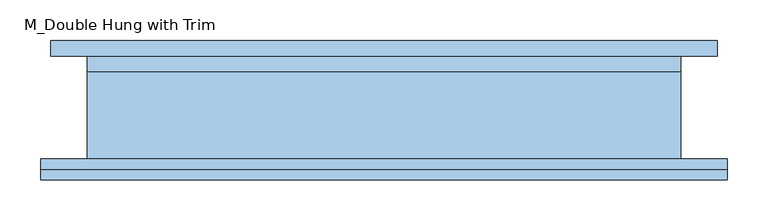
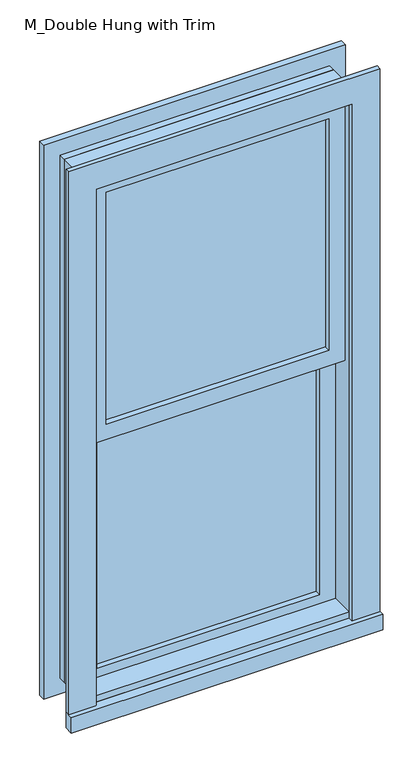
"""IFC4 building model written with IfcOpenShell, lengths in millimetres: window geometry, M_Double Hung with Trim."""

from ifc_helpers import new_model, si_unit, frame, origin, place, context, project, spatial, polyline, outline, extrude, source, transform, mapped, element, save


def m_double_hung_with_trim_aa4956d1(model_context):
    return source(origin(), model_context, "Body", "SweptSolid", [
        extrude(outline(polyline([(-301.625, 15.825), (-301.625, 28.525), (301.625, 28.525), (301.625, 15.825), (-301.625, 15.825)])), frame((0.0, 0.0, 628.65), z_axis=(0.0, 0.0, 1.0), x_axis=(1.0, 0.0, 0.0)), (0.0, 0.0, 1.0), 682.625),
        extrude(outline(polyline([(1355.725, -346.075), (584.2, -346.075), (584.2, 346.075), (1355.725, 346.075), (1355.725, -346.075)]), holes=[polyline([(1311.275, -301.625), (1311.275, 301.625), (628.65, 301.625), (628.65, -301.625), (1311.275, -301.625)])]), frame((0.0, -0.05, 0.0), z_axis=(0.0, 1.0, 0.0), x_axis=(0.0, 0.0, 1.0)), (0.0, 0.0, 1.0), 44.45),
        extrude(outline(polyline([(-422.275, -89.2), (-422.275, -63.5), (422.275, -63.5), (422.275, -89.2), (-422.275, -89.2)])), frame((0.0, 0.0, 539.75), z_axis=(0.0, 0.0, 1.0), x_axis=(1.0, 0.0, 0.0)), (0.0, 0.0, 1.0), 44.45),
        extrude(outline(polyline([(2139.95, -422.275), (539.75, -422.275), (539.75, 422.275), (2139.95, 422.275), (2139.95, -422.275)]), holes=[polyline([(2063.75, -346.075), (2063.75, 346.075), (584.2, 346.075), (584.2, -346.075), (2063.75, -346.075)])]), frame((0.0, -76.5, 0.0), z_axis=(0.0, 1.0, 0.0), x_axis=(0.0, 0.0, 1.0)), (0.0, 0.0, 1.0), 13.0),
        extrude(outline(polyline([(2127.25, 409.575), (2127.25, -409.575), (539.75, -409.575), (539.75, 409.575), (2127.25, 409.575)]), holes=[polyline([(2051.05, 333.375), (615.95, 333.375), (615.95, -333.375), (2051.05, -333.375), (2051.05, 333.375)])]), frame((0.0, 63.5, 0.0), z_axis=(0.0, 1.0, 0.0), x_axis=(0.0, 0.0, 1.0)), (0.0, 0.0, 1.0), 19.0),
        extrude(outline(polyline([(301.625, -15.925), (301.625, -28.625), (-301.625, -28.625), (-301.625, -15.925), (301.625, -15.925)])), frame((0.0, 0.0, 1355.725), z_axis=(0.0, 0.0, 1.0), x_axis=(1.0, 0.0, 0.0)), (0.0, 0.0, 1.0), 663.575),
        extrude(outline(polyline([(2063.75, -346.075), (1311.275, -346.075), (1311.275, 346.075), (2063.75, 346.075), (2063.75, -346.075)]), holes=[polyline([(2019.3, -301.625), (2019.3, 301.625), (1355.725, 301.625), (1355.725, -301.625), (2019.3, -301.625)])]), frame((0.0, -44.5, 0.0), z_axis=(0.0, 1.0, 0.0), x_axis=(0.0, 0.0, 1.0)), (0.0, 0.0, 1.0), 44.45),
        extrude(outline(polyline([(2082.8, -365.125), (584.2, -365.125), (584.2, 365.125), (2082.8, 365.125), (2082.8, -365.125)]), holes=[polyline([(2051.05, -333.375), (2051.05, 333.375), (615.95, 333.375), (615.95, -333.375), (2051.05, -333.375)])]), frame((0.0, 44.4, 0.0), z_axis=(0.0, 1.0, 0.0), x_axis=(0.0, 0.0, 1.0)), (0.0, 0.0, 1.0), 19.1),
        extrude(outline(polyline([(2082.8, 365.125), (2082.8, -365.125), (584.2, -365.125), (584.2, 365.125), (2082.8, 365.125)]), holes=[polyline([(2063.75, 346.075), (603.25, 346.075), (603.25, -346.075), (2063.75, -346.075), (2063.75, 346.075)])]), frame((0.0, -63.5, 0.0), z_axis=(0.0, 1.0, 0.0), x_axis=(0.0, 0.0, 1.0)), (0.0, 0.0, 1.0), 107.9),
    ])


if __name__ == "__main__":
    model = new_model("IFC4")
    model_context = context("Model", 3, world=origin())
    ifc_project = project(units=[si_unit("LENGTHUNIT", "METRE", prefix="MILLI")], contexts=[model_context])
    site = spatial("IfcSite", under=ifc_project)
    building = spatial("IfcBuilding", under=site)
    placement = place(None, origin())
    m_double_hung_with_trim_shape = m_double_hung_with_trim_aa4956d1(model_context)
    element("IfcWindow", 1, ObjectType="M_Double Hung with Trim : 2'  4 3/4\" x  4'  11\"", at=placement, inside=building, context=model_context, shape_type="MappedRepresentation", body=[
        mapped(m_double_hung_with_trim_shape, transform((0.0, 0.0, 0.0), x_axis=(1.0, 0.0, 0.0), y_axis=(0.0, 1.0, 0.0), z_axis=(0.0, 0.0, 1.0))),
    ])
    save(model, "model.ifc")

# Revit data of these elements
# Type "M_Double Hung with Trim : 2'  4 3/4\" x  4'  11\""
#   Type Mark = "73"
#   Construction Type Id = "GSP4R"
#   Analytic Construction = "1/8 in Pilkington single glazing"
#   Visual Light Transmittance = 0.9
#   Thermal Resistance (R) = 0.271106 (m²·K)/W
#   Solar Heat Gain Coefficient = 0.78
#   Heat Transfer Coefficient (U) = 3.6886 W/(m²·K)
#   Height = 4' - 11"
#   Default Sill Height = 1' - 11"
#   Trim Projection - Ext. = 0' - 0.51181"
#   Trim Projection - Int. = 0' - 0.74803"
#   Trim Width - Exterior = 0' - 3"
#   Trim Width - Interior = 0' - 3"
#   Width = 2' - 4 3/4"
#   Window Inset = 0' - 0.74803"
#   Glass Pane Material = EXISTING WINDOW
#   Sash = Trim
#   Trim Exterior Material = Trim
#   Trim Interior Material = Trim
#   Wall Closure = (empty or 0)
# Element 1 (IfcWindow, "M_Double Hung with Trim : 2'  4 3/4\" x  4'  11\"")
#   Materials on its faces: "Trim", "EXISTING WINDOW"
# Materials
#   "EXISTING WINDOW": class "Glass", colour RGB 218 227 224, transparency 0.85, Description = "Soda Lime Glass", Cost = 0
#   "Trim": class "Wood", colour RGB 250 251 245, transparency 0, Cost = 0
